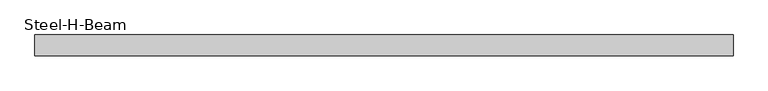
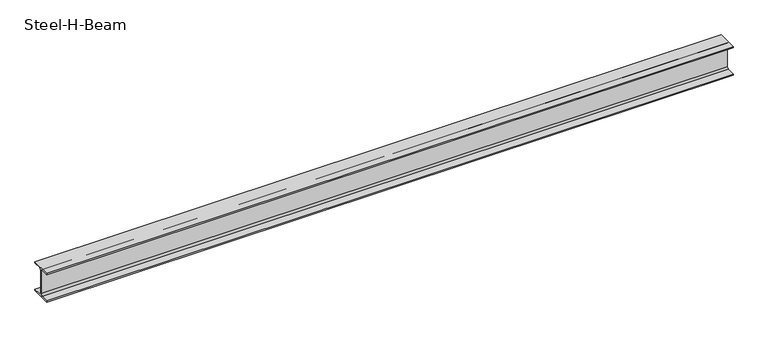
"""IFC4 building model written with IfcOpenShell, lengths in millimetres: beam geometry, Steel-H-Beam : BM121_H-294×200x8x12."""

import ifcopenshell
import ifcopenshell.guid

model = None  # the IFC model being written
_history = None  # IfcOwnerHistory: only IFC2X3 demands one
_inside = {}  # id of a spatial element -> (the spatial element, [elements in it])
_under = {}  # id of a project, library or spatial element -> (it, [spatial elements below it])
_declared = {}  # id of a project -> (the project, [libraries it declares])
_typed = {}  # id of a type object -> (the type object, [elements of that type])
_made_of = {}  # id of a material, layer set ... -> (it, [elements and type objects made of it])


def new_model(schema):
    """Start an empty IFC model of exactly this schema.

    Asked for "IFC4X3", IfcOpenShell would pick the latest addendum, in which some entities
    have other attributes; the version numbers below select the first issue.
    IFC2X3 requires an IfcOwnerHistory on every rooted entity: one is made here for all.
    """
    global model, _history
    if schema == "IFC4X3":
        model = ifcopenshell.file(schema_version=(4, 3, 0, 0))
    else:
        model = ifcopenshell.file(schema=schema)
    _inside.clear()
    _under.clear()
    _declared.clear()
    _typed.clear()
    _made_of.clear()
    _history = None
    if model.schema == "IFC2X3":
        org = make("IfcOrganization", Name="unknown")
        user = make(
            "IfcPersonAndOrganization",
            ThePerson=make("IfcPerson", FamilyName="unknown"),
            TheOrganization=org,
        )
        app = make(
            "IfcApplication",
            ApplicationDeveloper=org,
            Version="unknown",
            ApplicationFullName="unknown",
            ApplicationIdentifier="unknown",
        )
        _history = make(
            "IfcOwnerHistory",
            OwningUser=user,
            OwningApplication=app,
            ChangeAction="ADDED",
            CreationDate=0,
        )
    return model


def make(cls, **values):
    """One entity of the class cls with the attributes given. An attribute that is None is left unset."""
    return model.create_entity(
        cls, **{name: value for name, value in values.items() if value is not None}
    )


def rooted(cls, **values):
    """An entity with a GlobalId (a new one), such as an element, a storey or a relation."""
    return make(cls, GlobalId=ifcopenshell.guid.new(), OwnerHistory=_history, **values)


def si_unit(unit_type, name, prefix=None):
    """IfcSIUnit, for example si_unit("LENGTHUNIT", "METRE", prefix="MILLI")."""
    return make("IfcSIUnit", UnitType=unit_type, Prefix=prefix, Name=name)


def assignment(units):
    """IfcUnitAssignment: the units of a project."""
    return None if units is None else make("IfcUnitAssignment", Units=units)


def point(xyz):
    """IfcCartesianPoint."""
    return None if xyz is None else make("IfcCartesianPoint", Coordinates=xyz)


def direction(xyz):
    """IfcDirection."""
    return None if xyz is None else make("IfcDirection", DirectionRatios=xyz)


def frame(location, z_axis=None, x_axis=None):
    """IfcAxis2Placement3D, a coordinate frame: its origin and axes. An axis left out is left unset."""
    return make(
        "IfcAxis2Placement3D",
        Location=point(location),
        Axis=direction(z_axis),
        RefDirection=direction(x_axis),
    )


def frame_2d(location, x_axis=None):
    """IfcAxis2Placement2D, a coordinate frame in the plane: its origin and x axis."""
    return make(
        "IfcAxis2Placement2D", Location=point(location), RefDirection=direction(x_axis)
    )


def origin():
    """The frame at (0, 0, 0) with its axes left unset."""
    return frame((0.0, 0.0, 0.0))


def place(relative_to, where):
    """IfcLocalPlacement: puts the frame where relative to a parent placement (None: the world)."""
    return make(
        "IfcLocalPlacement", PlacementRelTo=relative_to, RelativePlacement=where
    )


def context(
    kind, dimensions, precision=None, world=None, true_north=None, identifier=None
):
    """IfcGeometricRepresentationContext, for example the 3D "Model" context."""
    return make(
        "IfcGeometricRepresentationContext",
        ContextIdentifier=identifier,
        ContextType=kind,
        CoordinateSpaceDimension=dimensions,
        Precision=precision,
        WorldCoordinateSystem=world,
        TrueNorth=true_north,
    )


def project(units=None, contexts=None):
    """IfcProject with its units and contexts."""
    return rooted(
        "IfcProject",
        Name="project",
        RepresentationContexts=contexts,
        UnitsInContext=assignment(units),
    )


def spatial(cls, under=None, at=None, **own):
    """A site, building, storey or space (cls), placed at a placement, below another one or the project."""
    s = rooted(cls, ObjectPlacement=at, **own)
    if under is not None:
        _under.setdefault(under.id(), (under, []))[1].append(s)
    return s


def polyline(points):
    """IfcPolyline through the points."""
    return make("IfcPolyline", Points=[point(p) for p in points])


def circle_curve(where, radius):
    """IfcCircle in the frame where."""
    return make("IfcCircle", Position=where, Radius=radius)


def trimmed(basis, trim1, trim2, sense, master):
    """IfcTrimmedCurve: the piece of a basis curve between two trims."""
    return make(
        "IfcTrimmedCurve",
        BasisCurve=basis,
        Trim1=trim1,
        Trim2=trim2,
        SenseAgreement=sense,
        MasterRepresentation=master,
    )


def segment(curve, same_sense, transition):
    """IfcCompositeCurveSegment."""
    return make(
        "IfcCompositeCurveSegment",
        Transition=transition,
        SameSense=same_sense,
        ParentCurve=curve,
    )


def composite_curve(segments, self_intersect=None):
    """IfcCompositeCurve: segments joined end to end."""
    return make("IfcCompositeCurve", Segments=segments, SelfIntersect=self_intersect)


def outline(outer, holes=None, kind="AREA"):
    """IfcArbitraryClosedProfileDef: a profile drawn as a closed curve; with holes, ...WithVoids."""
    if holes is None:
        return make("IfcArbitraryClosedProfileDef", ProfileType=kind, OuterCurve=outer)
    return make(
        "IfcArbitraryProfileDefWithVoids",
        ProfileType=kind,
        OuterCurve=outer,
        InnerCurves=holes,
    )


def extrude(swept, where, along, depth):
    """IfcExtrudedAreaSolid: the profile swept, set in the frame where, extruded along a direction by depth."""
    return make(
        "IfcExtrudedAreaSolid",
        SweptArea=swept,
        Position=where,
        ExtrudedDirection=direction(along),
        Depth=depth,
    )


def shape(context_of_items, identifier, shape_type, items):
    """IfcShapeRepresentation: the items that make up one representation, for example the "Body"."""
    return make(
        "IfcShapeRepresentation",
        ContextOfItems=context_of_items,
        RepresentationIdentifier=identifier,
        RepresentationType=shape_type,
        Items=items,
    )


def source(mapping_origin, context_of_items, identifier, shape_type, items):
    """IfcRepresentationMap: a shape defined once, which mapped items show again and again."""
    return make(
        "IfcRepresentationMap",
        MappingOrigin=mapping_origin,
        MappedRepresentation=shape(context_of_items, identifier, shape_type, items),
    )


def transform(
    local_origin,
    x_axis=None,
    y_axis=None,
    z_axis=None,
    scale=None,
    scale2=None,
    scale3=None,
    uniform=True,
):
    """IfcCartesianTransformationOperator3D, or its non-uniform kind. x_axis, y_axis, z_axis: its Axis1, 2, 3."""
    if uniform:
        return make(
            "IfcCartesianTransformationOperator3D",
            Axis1=direction(x_axis),
            Axis2=direction(y_axis),
            LocalOrigin=point(local_origin),
            Scale=scale,
            Axis3=direction(z_axis),
        )
    return make(
        "IfcCartesianTransformationOperator3DnonUniform",
        Axis1=direction(x_axis),
        Axis2=direction(y_axis),
        LocalOrigin=point(local_origin),
        Scale=scale,
        Axis3=direction(z_axis),
        Scale2=scale2,
        Scale3=scale3,
    )


def mapped(mapping_source, mapping_target):
    """IfcMappedItem: shows the shape of a source again, moved by a transform."""
    return make(
        "IfcMappedItem", MappingSource=mapping_source, MappingTarget=mapping_target
    )


def made_of(thing, what):
    """Note that an element or type object is made of a material, layer set ...; save() writes the relation."""
    if what is not None:
        _made_of.setdefault(what.id(), (what, []))[1].append(thing)
    return thing


def element(
    cls,
    number,
    at=None,
    inside=None,
    cuts=None,
    type_object=None,
    material=None,
    context=None,
    identifier="Body",
    shape_type=None,
    held_by="IfcProductDefinitionShape",
    body=None,
    shapes=None,
    **own,
):
    """One element of the class cls, such as IfcWall. Its Tag is "e" and its number.

    at: its placement. inside: the storey or other place that contains it. cuts: it is an
    opening in that element (IfcRelVoidsElement). A single representation is given by context,
    identifier, shape_type and body (its items); several are given by shapes. held_by: the class
    of the entity that holds the representations. save() writes the other relations.
    """
    e = rooted(cls, Tag="e%d" % number, ObjectPlacement=at, **own)
    if body is not None:
        shapes = [shape(context, identifier, shape_type, body)]
    if shapes is not None:
        e.Representation = make(held_by, Representations=shapes)
    if inside is not None:
        _inside.setdefault(inside.id(), (inside, []))[1].append(e)
    if cuts is not None:
        rooted(
            "IfcRelVoidsElement", RelatingBuildingElement=cuts, RelatedOpeningElement=e
        )
    if type_object is not None:
        _typed.setdefault(type_object.id(), (type_object, []))[1].append(e)
    return made_of(e, material)


def aggregate(whole, parts):
    """IfcRelAggregates: a whole, such as a stair, and the parts it consists of."""
    return rooted("IfcRelAggregates", RelatingObject=whole, RelatedObjects=parts)


def save(model, path):
    """Write the relations noted so far, then the file.

    IfcRelAggregates (storeys below a building ...), IfcRelContainedInSpatialStructure (elements
    in a storey), IfcRelDefinesByType, IfcRelAssociatesMaterial and IfcRelDeclares: one each for
    every whole, place, type object, material and project.
    """
    for whole, parts in _under.values():
        aggregate(whole, parts)
    for where, things in _inside.values():
        rooted(
            "IfcRelContainedInSpatialStructure",
            RelatedElements=things,
            RelatingStructure=where,
        )
    for kind, things in _typed.values():
        rooted("IfcRelDefinesByType", RelatedObjects=things, RelatingType=kind)
    for what, things in _made_of.values():
        rooted("IfcRelAssociatesMaterial", RelatedObjects=things, RelatingMaterial=what)
    for by, libraries in _declared.values():
        rooted("IfcRelDeclares", RelatingContext=by, RelatedDefinitions=libraries)
    model.write(path)


def steel_h_beam_3e669b2c(model_context):
    return source(origin(), model_context, "Body", "SweptSolid", [
        extrude(outline(composite_curve([segment(polyline([(100.0, -135.0), (100.0, -147.0), (-100.0, -147.0), (-100.0, -135.0), (-22.0, -135.0)]), True, "CONTINUOUS"), segment(trimmed(circle_curve(frame_2d((-22.0, -117.0)), 18.0), [point((-22.0, -135.0))], [point((-4.0, -117.0))], True, "CARTESIAN"), True, "CONTINUOUS"), segment(polyline([(-4.0, -117.0), (-4.0, 117.0)]), True, "CONTINUOUS"), segment(trimmed(circle_curve(frame_2d((-22.0, 117.0)), 18.0), [point((-4.0, 117.0))], [point((-22.0, 135.0))], True, "CARTESIAN"), True, "CONTINUOUS"), segment(polyline([(-22.0, 135.0), (-100.0, 135.0), (-100.0, 147.0), (100.0, 147.0), (100.0, 135.0), (22.0, 135.0)]), True, "CONTINUOUS"), segment(trimmed(circle_curve(frame_2d((22.0, 117.0)), 18.0), [point((22.0, 135.0))], [point((4.0, 117.0))], True, "CARTESIAN"), True, "CONTINUOUS"), segment(polyline([(4.0, 117.0), (4.0, -117.0)]), True, "CONTINUOUS"), segment(trimmed(circle_curve(frame_2d((22.0, -117.0)), 18.0), [point((4.0, -117.0))], [point((22.0, -135.0))], True, "CARTESIAN"), True, "CONTINUOUS"), segment(polyline([(22.0, -135.0), (100.0, -135.0)]), True, "CONTINUOUS")], self_intersect=False)), frame((-3500.0, 0.0, 0.0), z_axis=(1.0, 0.0, 0.0), x_axis=(0.0, 1.0, 0.0)), (0.0, 0.0, 1.0), 6687.2337007),
    ])


if __name__ == "__main__":
    model = new_model("IFC4")
    model_context = context("Model", 3, world=origin())
    ifc_project = project(units=[si_unit("LENGTHUNIT", "METRE", prefix="MILLI")], contexts=[model_context])
    site = spatial("IfcSite", under=ifc_project)
    building = spatial("IfcBuilding", under=site)
    placement = place(None, origin())
    steel_h_beam_shape = steel_h_beam_3e669b2c(model_context)
    element("IfcBeam", 1, ObjectType="Steel-H-Beam : BM121_H-294×200x8x12", at=placement, inside=building, context=model_context, shape_type="MappedRepresentation", body=[
        mapped(steel_h_beam_shape, transform((0.0, 0.0, 0.0), x_axis=(1.0, 0.0, 0.0), y_axis=(0.0, 1.0, 0.0), z_axis=(0.0, 0.0, 1.0))),
    ])
    save(model, "model.ifc")

# Revit data of these elements
# Type "Steel-H-Beam : BM121_H-294×200x8x12"
#   Surface Area = 1.3411 m²/m
#   Section Area = 72.3812 cm²
#   Mass per Unit Length = 56.8193 kg/m
#   Length [instance default] = 3000 mm
#   B = 200 mm
#   H = 294 mm
#   r = 18 mm
#   tw = 8 mm
#   tf = 12 mm
#   hec_material4 [instance default] = none
#   hec_material3 [instance default] = none
#   hec_material2 [instance default] = none
#   hec_material1 [instance default] = none
#   Structural Material [instance default] = Steel, 45-345
#   Assembly Code = ""
# Element 1 (IfcBeam, "Steel-H-Beam : BM121_H-294×200x8x12")
#   hec_material3 = F01AC000-00002_Building/Shelter Fire Proofing Work_Intumescent Coating Type_1 hr. rating (UL 1709))
#   hec_material2 = S01AA010-00002_Main Steel Structure Fabrication Work_Shelter/Building_Steel Painting/Coating_for Fireproofed Steel Surface, Surface Preparation & Primer Coat
#   hec_material1 = S03AA028-00001_Main Steel Structure Erection Work_Shelter/Building_Medium Steel
#   Structural Material = S01AA002-00001_Main Steel Structure Fabrication Work_Shelter/Building_Medium Steel - Standard
#   Materials on its faces: "S01AA002-00001_Main Steel Structure Fabrication Work_Shelter/Building_Medium Steel - Standard"
# Materials
#   "Steel, 45-345": class "Metal", colour RGB 189 187 185, transparency 0, Description = "Steel 345 MPa", Cost = 0
#   "S01AA002-00001_Main Steel Structure Fabrication Work_Shelter/Building_Medium Steel - Standard": class "Metal", colour RGB 120 120 120, transparency 0, Comments = "(90KG/M>Weight≥30KG/M)", Description = "Structural steel 50ksi", W00) Work Master Code = "S01AA002-0001", W01) Work Master_Lv1 = "Main Steel Structure Fabrication Work", W02) Work Master_Lv2 = "Shelter/Building", W03) Work Master_Spec.1 = "Medium Steel - Standard (90KG/M>Weight≥30KG/M)", Cost = 0
#   "F01AC000-00002_Building/Shelter Fire Proofing Work_Intumescent Coating Type_1 hr. rating (UL 1709))": class "Metal", colour RGB 255 128 128, transparency 0, Description = "Paint finished steel", W00) Work Master Code = "F01AC000-00002", W01) Work Master_Lv1 = "Building/Shelter Fire Proofing Work", W02) Work Master_Lv2 = "Intumescent Coating Type", W03) Work Master_Spec.1 = "1 hr. rating (UL 1709)", Cost = 0
#   "S01AA010-00002_Main Steel Structure Fabrication Work_Shelter/Building_Steel Painting/Coating_for Fireproofed Steel Surface, Surface Preparation & Primer Coat": class "Metal", colour RGB 120 120 120, transparency 0, Description = "Paint finished steel", W00) Work Master Code = "SS01AA010-00002", W01) Work Master_Lv1 = "Main Steel Structure Fabrication Work", W02) Work Master_Lv2 = "Shelter/Building", W03) Work Master_Spec.1 = "Steel Painting/Coating", W04) Work Master_Spec.2 = "for Fireproofed Steel Surface, Surface Preparation & Primer Coat", Cost = 0
#   "S03AA028-00001_Main Steel Structure Erection Work_Shelter/Building_Medium Steel": class "Metal", colour RGB 120 120 120, transparency 0, Comments = "(90KG/M>Weight≥30KG/M)", Description = "Structural steel 50ksi", W00) Work Master Code = "S03AA028-0001", W01) Work Master_Lv1 = "Main Steel Structure Erection Work", W02) Work Master_Lv2 = "Shelter/Building", W03) Work Master_Spec.1 = "Medium Steel (90KG/M>Weight≥30KG/M)", Cost = 0
